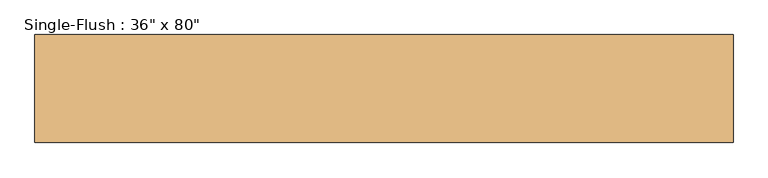
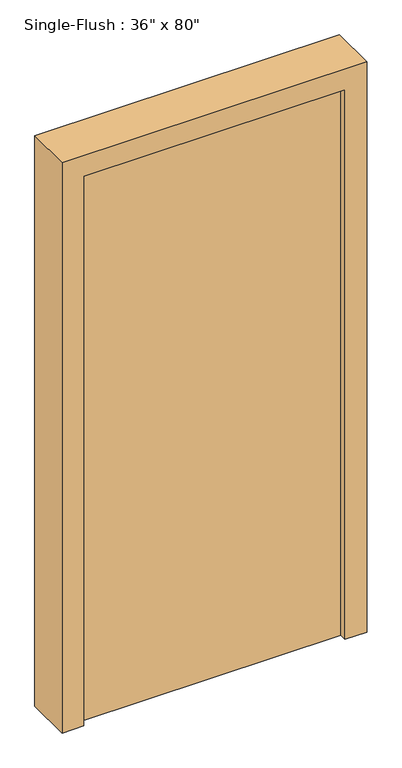
"""IFC4 building model written with IfcOpenShell, lengths in millimetres: door geometry."""

from ifc_helpers import new_model, si_unit, frame, origin, origin_with_axes, place, context, project, spatial, polyline, outline, extrude, source, transform, mapped, element, save


def door_3f9ad012(model_context):
    return source(origin(), model_context, "Body", "SweptSolid", [
        extrude(outline(polyline([(2108.2, 533.4), (2108.2, -533.4), (0.0, -533.4), (0.0, -457.2), (2032.0, -457.2), (2032.0, 457.2), (0.0, 457.2), (0.0, 533.4), (2108.2, 533.4)])), frame((0.0, -82.55, 0.0), z_axis=(0.0, 1.0, 0.0), x_axis=(0.0, 0.0, 1.0)), (0.0, 0.0, 1.0), 165.1),
        extrude(outline(polyline([(457.2, -6.35), (457.2, -57.15), (-457.2, -57.15), (-457.2, -6.35), (457.2, -6.35)])), origin_with_axes(), (0.0, 0.0, 1.0), 2032.0),
    ])


if __name__ == "__main__":
    model = new_model("IFC4")
    model_context = context("Model", 3, world=origin())
    ifc_project = project(units=[si_unit("LENGTHUNIT", "METRE", prefix="MILLI")], contexts=[model_context])
    site = spatial("IfcSite", under=ifc_project)
    building = spatial("IfcBuilding", under=site)
    placement = place(None, origin())
    door_shape = door_3f9ad012(model_context)
    element("IfcDoor", 1, ObjectType="Single-Flush : 36\" x 80\"", at=placement, inside=building, context=model_context, shape_type="MappedRepresentation", body=[
        mapped(door_shape, transform((0.0, 0.0, 0.0), x_axis=(1.0, 0.0, 0.0), y_axis=(0.0, 1.0, 0.0), z_axis=(0.0, 0.0, 1.0))),
    ])
    save(model, "model.ifc")

# Revit data of these elements
# Type "Single-Flush : 36\" x 80\""
#   Type Mark = "6"
#   OD_DS_Door_Material = "T.B.D."
#   OD_DS_Door_Type = "SWING"
#   OD_DS_Lockset = "PRIVACY LOCK"
#   Assembly Code = "C1020"
#   Analytic Construction = "<None>"
#   Thickness = 0' - 2"
#   RO Offset = 0' - 0 1/4"
#   Height = 6' - 8"
#   Trim Projection Ext = 0' - 1"
#   Trim Projection Int = 0' - 1"
#   Trim Width = 0' - 3"
#   Width = 3' - 0"
#   Door Material = Closet_1
#   Frame Material = Closet_1
#   Function = (empty or 0)
#   Wall Closure = (empty or 0)
# Element 1 (IfcDoor, "Single-Flush : 36\" x 80\"")
#   Materials on its faces: "Closet_1"
# Materials
#   "Closet_1": class "Paint", colour RGB 200 194 183, transparency 0, Cost = 0
